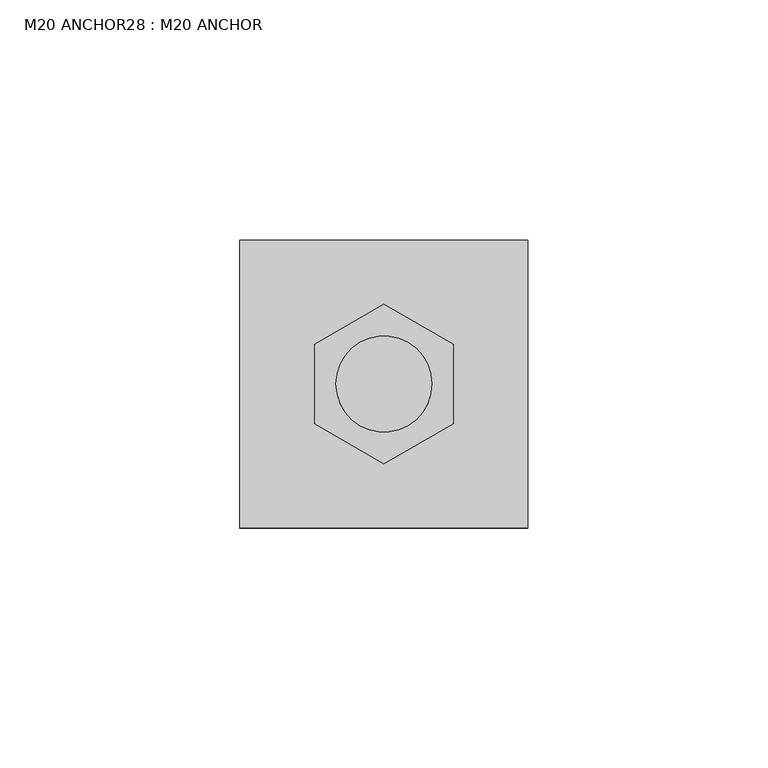
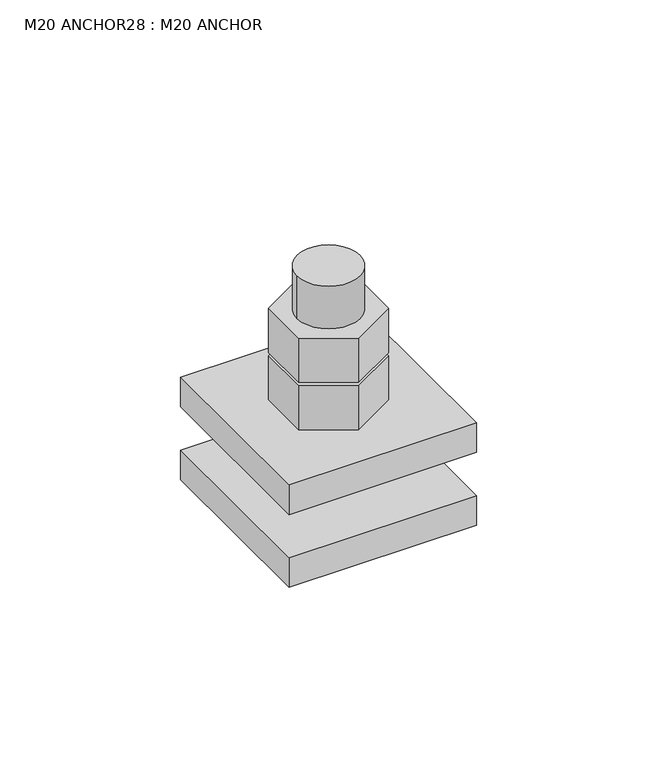
"""IFC4 building model written with IfcOpenShell, lengths in millimetres: fastener geometry, M20 ANCHOR28 : M20 ANCHOR."""

from ifc_helpers import new_model, si_unit, point, frame, frame_2d, origin, place, context, project, spatial, polyline, circle_curve, trimmed, segment, composite_curve, outline, extrude, source, transform, mapped, element, save


def m20_anchor28_m20_anchor_5836d441(model_context):
    return source(origin(), model_context, "Body", "SweptSolid", [
        extrude(outline(polyline([(-30672.4939916, -7426.8093347), (-30686.9021106, -7435.1278661), (-30701.3102297, -7426.8093347), (-30701.3102297, -7410.1722719), (-30686.9021106, -7401.8537405), (-30672.4939916, -7410.1722719), (-30672.4939916, -7426.8093347)]), holes=[composite_curve([segment(trimmed(circle_curve(frame_2d((-30686.9021106, -7418.4908033)), 10.0), [point((-30696.9021106, -7418.4908033))], [point((-30676.9021106, -7418.4908033))], True, "CARTESIAN"), True, "CONTINUOUS"), segment(trimmed(circle_curve(frame_2d((-30686.9021106, -7418.4908033)), 10.0), [point((-30676.9021106, -7418.4908033))], [point((-30696.9021106, -7418.4908033))], True, "CARTESIAN"), True, "CONTINUOUS")], self_intersect=False)]), frame((0.0, 0.0, 240.605), z_axis=(0.0, 0.0, 1.0), x_axis=(1.0, 0.0, 0.0)), (0.0, 0.0, 1.0), 15.0),
        extrude(outline(polyline([(-30672.4939916, -7426.8093347), (-30686.9021106, -7435.1278661), (-30701.3102297, -7426.8093347), (-30701.3102297, -7410.1722719), (-30686.9021106, -7401.8537405), (-30672.4939916, -7410.1722719), (-30672.4939916, -7426.8093347)]), holes=[composite_curve([segment(trimmed(circle_curve(frame_2d((-30686.9021106, -7418.4908033)), 10.0), [point((-30696.9021106, -7418.4908033))], [point((-30676.9021106, -7418.4908033))], True, "CARTESIAN"), True, "CONTINUOUS"), segment(trimmed(circle_curve(frame_2d((-30686.9021106, -7418.4908033)), 10.0), [point((-30676.9021106, -7418.4908033))], [point((-30696.9021106, -7418.4908033))], True, "CARTESIAN"), True, "CONTINUOUS")], self_intersect=False)]), frame((0.0, 0.0, 224.605), z_axis=(0.0, 0.0, 1.0), x_axis=(1.0, 0.0, 0.0)), (0.0, 0.0, 1.0), 15.0),
        extrude(outline(composite_curve([segment(trimmed(circle_curve(frame_2d((-30686.9021106, -7418.4908033)), 10.0), [point((-30696.9021106, -7418.4908033))], [point((-30676.9021106, -7418.4908033))], False, "CARTESIAN"), True, "CONTINUOUS"), segment(trimmed(circle_curve(frame_2d((-30686.9021106, -7418.4908033)), 10.0), [point((-30676.9021106, -7418.4908033))], [point((-30696.9021106, -7418.4908033))], False, "CARTESIAN"), True, "CONTINUOUS")], self_intersect=False)), frame((0.0, 0.0, 190.0), z_axis=(0.0, 0.0, 1.0), x_axis=(1.0, 0.0, 0.0)), (0.0, 0.0, 1.0), 80.0),
        extrude(outline(polyline([(-30656.9021106, -7448.4908033), (-30716.9021106, -7448.4908033), (-30716.9021106, -7388.4908033), (-30656.9021106, -7388.4908033), (-30656.9021106, -7448.4908033)]), holes=[composite_curve([segment(trimmed(circle_curve(frame_2d((-30686.9021106, -7418.4908033)), 11.0), [point((-30697.9021106, -7418.4908033))], [point((-30675.9021106, -7418.4908033))], True, "CARTESIAN"), True, "CONTINUOUS"), segment(trimmed(circle_curve(frame_2d((-30686.9021106, -7418.4908033)), 11.0), [point((-30675.9021106, -7418.4908033))], [point((-30697.9021106, -7418.4908033))], True, "CARTESIAN"), True, "CONTINUOUS")], self_intersect=False)]), frame((0.0, 0.0, 190.0), z_axis=(0.0, 0.0, 1.0), x_axis=(1.0, 0.0, 0.0)), (0.0, 0.0, 1.0), 10.0),
        extrude(outline(polyline([(-30656.9021106, -7448.4908033), (-30716.9021106, -7448.4908033), (-30716.9021106, -7388.4908033), (-30656.9021106, -7388.4908033), (-30656.9021106, -7448.4908033)]), holes=[composite_curve([segment(trimmed(circle_curve(frame_2d((-30686.9021106, -7418.4908033)), 11.0), [point((-30697.9021106, -7418.4908033))], [point((-30675.9021106, -7418.4908033))], True, "CARTESIAN"), True, "CONTINUOUS"), segment(trimmed(circle_curve(frame_2d((-30686.9021106, -7418.4908033)), 11.0), [point((-30675.9021106, -7418.4908033))], [point((-30697.9021106, -7418.4908033))], True, "CARTESIAN"), True, "CONTINUOUS")], self_intersect=False)]), frame((0.0, 0.0, 214.605), z_axis=(0.0, 0.0, 1.0), x_axis=(1.0, 0.0, 0.0)), (0.0, 0.0, 1.0), 10.0),
    ])


if __name__ == "__main__":
    model = new_model("IFC4")
    model_context = context("Model", 3, world=origin())
    ifc_project = project(units=[si_unit("LENGTHUNIT", "METRE", prefix="MILLI")], contexts=[model_context])
    site = spatial("IfcSite", under=ifc_project)
    building = spatial("IfcBuilding", under=site)
    placement = place(None, origin())
    m20_anchor28_m20_anchor_shape = m20_anchor28_m20_anchor_5836d441(model_context)
    element("IfcFastener", 1, ObjectType="M20 ANCHOR28 : M20 ANCHOR", at=placement, inside=building, context=model_context, shape_type="MappedRepresentation", body=[
        mapped(m20_anchor28_m20_anchor_shape, transform((0.0, 0.0, 0.0), x_axis=(1.0, 0.0, 0.0), y_axis=(0.0, 1.0, 0.0), z_axis=(0.0, 0.0, 1.0))),
    ])
    save(model, "model.ifc")
